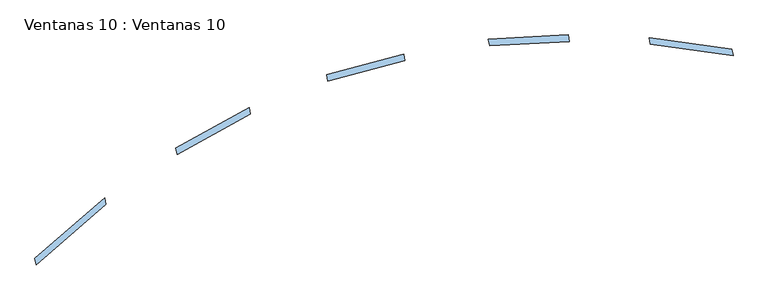
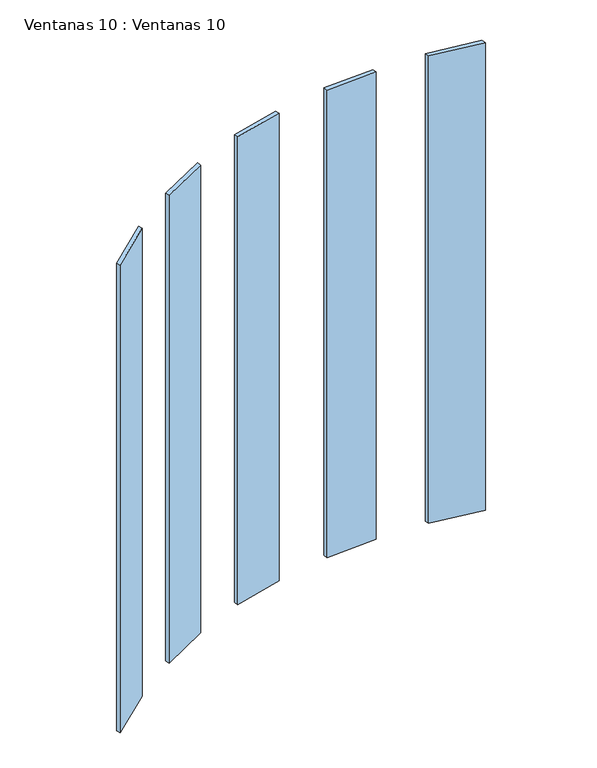
"""IFC4 building model written with IfcOpenShell, lengths in millimetres: window geometry, Ventanas 10 : Ventanas 10."""

from ifc_helpers import new_model, si_unit, frame, origin, place, context, project, spatial, polyline, outline, extrude, source, transform, mapped, element, save


def ventanas_10_ventanas_10_9fe3d7ef(model_context):
    return source(origin(), model_context, "Body", "SweptSolid", [
        extrude(outline(polyline([(-11934.3246908, -1437.332243), (-11930.8517273, -1457.0283981), (-12138.9540696, -1637.9290043), (-12142.4270331, -1618.2328493), (-11934.3246908, -1437.332243)])), frame((0.0, 0.0, 6537.7853888), z_axis=(0.0, 0.0, 1.0), x_axis=(1.0, 0.0, 0.0)), (0.0, 0.0, 1.0), 2321.1357802),
        extrude(outline(polyline([(-11503.9256181, -1167.8615111), (-11500.4526546, -1187.5576662), (-11719.0837315, -1308.7468511), (-11722.556695, -1289.050696), (-11503.9256181, -1167.8615111)])), frame((0.0, 0.0, 6537.7853888), z_axis=(0.0, 0.0, 1.0), x_axis=(1.0, 0.0, 0.0)), (0.0, 0.0, 1.0), 2321.1357802),
        extrude(outline(polyline([(-11044.0022823, -1008.5069856), (-11040.5293187, -1028.2031406), (-11269.701687, -1089.6096916), (-11273.1746505, -1069.9135366), (-11044.0022823, -1008.5069856)])), frame((0.0, 0.0, 6537.7853888), z_axis=(0.0, 0.0, 1.0), x_axis=(1.0, 0.0, 0.0)), (0.0, 0.0, 1.0), 2321.1357802),
        extrude(outline(polyline([(-10554.0397519, -951.5816665), (-10550.5667884, -971.2778216), (-10788.369278, -983.740522), (-10791.8422416, -964.0443669), (-10554.0397519, -951.5816665)])), frame((0.0, 0.0, 6537.7853888), z_axis=(0.0, 0.0, 1.0), x_axis=(1.0, 0.0, 0.0)), (0.0, 0.0, 1.0), 2321.1357802),
        extrude(outline(polyline([(-10066.4541981, -994.6014799), (-10062.9812346, -1014.297635), (-10309.0798388, -979.7107317), (-10312.5528023, -960.0145767), (-10066.4541981, -994.6014799)])), frame((0.0, 0.0, 6537.7853888), z_axis=(0.0, 0.0, 1.0), x_axis=(1.0, 0.0, 0.0)), (0.0, 0.0, 1.0), 2321.1357802),
    ])


if __name__ == "__main__":
    model = new_model("IFC4")
    model_context = context("Model", 3, world=origin())
    ifc_project = project(units=[si_unit("LENGTHUNIT", "METRE", prefix="MILLI")], contexts=[model_context])
    site = spatial("IfcSite", under=ifc_project)
    building = spatial("IfcBuilding", under=site)
    placement = place(None, origin())
    ventanas_10_ventanas_10_shape = ventanas_10_ventanas_10_9fe3d7ef(model_context)
    element("IfcWindow", 1, ObjectType="Ventanas 10 : Ventanas 10", at=placement, inside=building, context=model_context, shape_type="MappedRepresentation", body=[
        mapped(ventanas_10_ventanas_10_shape, transform((0.0, 0.0, 0.0), x_axis=(1.0, 0.0, 0.0), y_axis=(0.0, 1.0, 0.0), z_axis=(0.0, 0.0, 1.0))),
    ])
    save(model, "model.ifc")

# Revit data of these elements
# Type "Ventanas 10 : Ventanas 10"
#   Type Mark = "36"
# Element 1 (IfcWindow, "Ventanas 10 : Ventanas 10")
#   Materials on its faces: "VIDRIO"
# Materials
#   "VIDRIO": class "Genérico", colour RGB 120 120 120, transparency 0, Cost = 0
